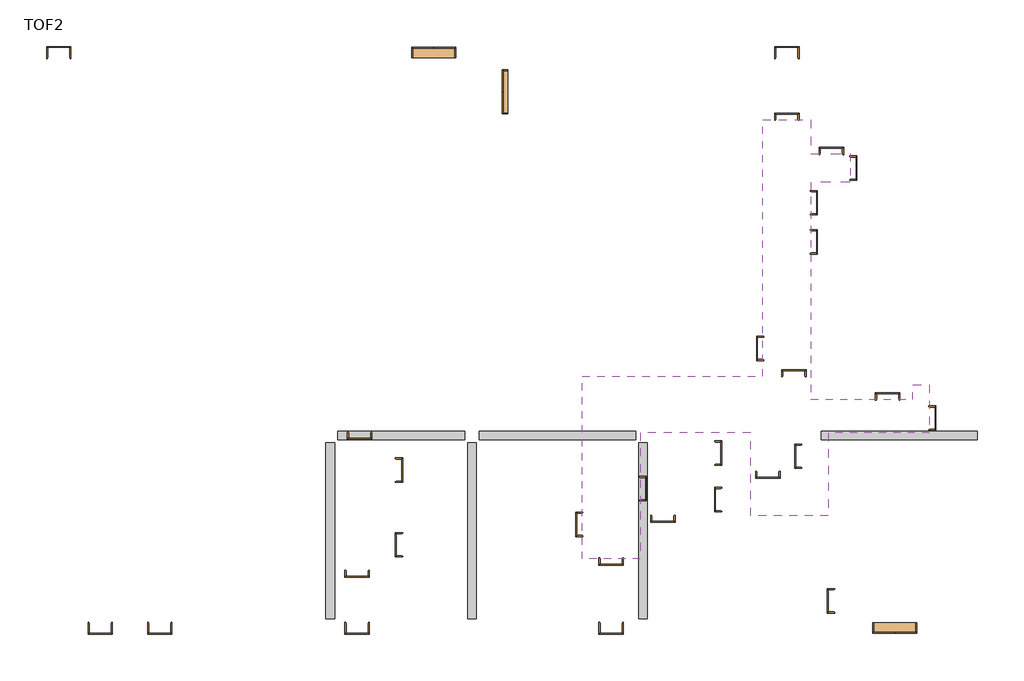
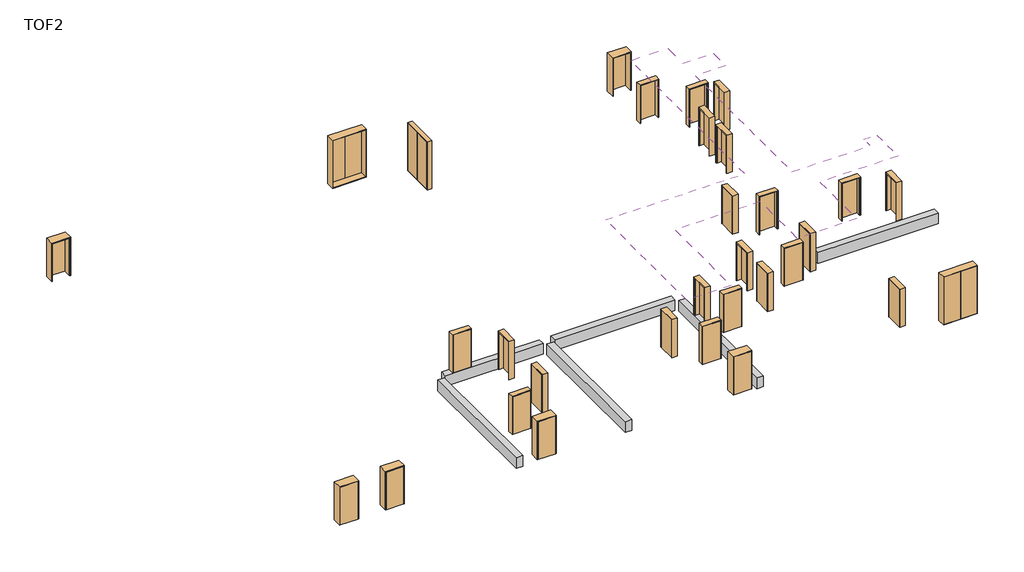
# One storey: 31 doors, 6 beams, 1 covering.
"""IFC4 building model written with IfcOpenShell, lengths in millimetres."""

import ifcopenshell
import ifcopenshell.guid

model = None  # the IFC model being written
_history = None  # IfcOwnerHistory: only IFC2X3 demands one
_inside = {}  # id of a spatial element -> (the spatial element, [elements in it])
_under = {}  # id of a project, library or spatial element -> (it, [spatial elements below it])
_declared = {}  # id of a project -> (the project, [libraries it declares])
_typed = {}  # id of a type object -> (the type object, [elements of that type])
_made_of = {}  # id of a material, layer set ... -> (it, [elements and type objects made of it])


def new_model(schema):
    """Start an empty IFC model of exactly this schema.

    Asked for "IFC4X3", IfcOpenShell would pick the latest addendum, in which some entities
    have other attributes; the version numbers below select the first issue.
    IFC2X3 requires an IfcOwnerHistory on every rooted entity: one is made here for all.
    """
    global model, _history
    if schema == "IFC4X3":
        model = ifcopenshell.file(schema_version=(4, 3, 0, 0))
    else:
        model = ifcopenshell.file(schema=schema)
    _inside.clear()
    _under.clear()
    _declared.clear()
    _typed.clear()
    _made_of.clear()
    _history = None
    if model.schema == "IFC2X3":
        org = make("IfcOrganization", Name="unknown")
        user = make(
            "IfcPersonAndOrganization",
            ThePerson=make("IfcPerson", FamilyName="unknown"),
            TheOrganization=org,
        )
        app = make(
            "IfcApplication",
            ApplicationDeveloper=org,
            Version="unknown",
            ApplicationFullName="unknown",
            ApplicationIdentifier="unknown",
        )
        _history = make(
            "IfcOwnerHistory",
            OwningUser=user,
            OwningApplication=app,
            ChangeAction="ADDED",
            CreationDate=0,
        )
    return model


def make(cls, **values):
    """One entity of the class cls with the attributes given. An attribute that is None is left unset."""
    return model.create_entity(
        cls, **{name: value for name, value in values.items() if value is not None}
    )


def rooted(cls, **values):
    """An entity with a GlobalId (a new one), such as an element, a storey or a relation."""
    return make(cls, GlobalId=ifcopenshell.guid.new(), OwnerHistory=_history, **values)


def si_unit(unit_type, name, prefix=None):
    """IfcSIUnit, for example si_unit("LENGTHUNIT", "METRE", prefix="MILLI")."""
    return make("IfcSIUnit", UnitType=unit_type, Prefix=prefix, Name=name)


def assignment(units):
    """IfcUnitAssignment: the units of a project."""
    return None if units is None else make("IfcUnitAssignment", Units=units)


def point(xyz):
    """IfcCartesianPoint."""
    return None if xyz is None else make("IfcCartesianPoint", Coordinates=xyz)


def direction(xyz):
    """IfcDirection."""
    return None if xyz is None else make("IfcDirection", DirectionRatios=xyz)


def frame(location, z_axis=None, x_axis=None):
    """IfcAxis2Placement3D, a coordinate frame: its origin and axes. An axis left out is left unset."""
    return make(
        "IfcAxis2Placement3D",
        Location=point(location),
        Axis=direction(z_axis),
        RefDirection=direction(x_axis),
    )


def origin():
    """The frame at (0, 0, 0) with its axes left unset."""
    return frame((0.0, 0.0, 0.0))


def origin_with_axes():
    """The frame at (0, 0, 0) with the z axis (0, 0, 1) and the x axis (1, 0, 0) written out."""
    return frame((0.0, 0.0, 0.0), z_axis=(0.0, 0.0, 1.0), x_axis=(1.0, 0.0, 0.0))


def place(relative_to, where):
    """IfcLocalPlacement: puts the frame where relative to a parent placement (None: the world)."""
    return make(
        "IfcLocalPlacement", PlacementRelTo=relative_to, RelativePlacement=where
    )


def context(
    kind, dimensions, precision=None, world=None, true_north=None, identifier=None
):
    """IfcGeometricRepresentationContext, for example the 3D "Model" context."""
    return make(
        "IfcGeometricRepresentationContext",
        ContextIdentifier=identifier,
        ContextType=kind,
        CoordinateSpaceDimension=dimensions,
        Precision=precision,
        WorldCoordinateSystem=world,
        TrueNorth=true_north,
    )


def project(units=None, contexts=None):
    """IfcProject with its units and contexts."""
    return rooted(
        "IfcProject",
        Name="project",
        RepresentationContexts=contexts,
        UnitsInContext=assignment(units),
    )


def spatial(cls, under=None, at=None, **own):
    """A site, building, storey or space (cls), placed at a placement, below another one or the project."""
    s = rooted(cls, ObjectPlacement=at, **own)
    if under is not None:
        _under.setdefault(under.id(), (under, []))[1].append(s)
    return s


def polyline(points):
    """IfcPolyline through the points."""
    return make("IfcPolyline", Points=[point(p) for p in points])


def outline(outer, holes=None, kind="AREA"):
    """IfcArbitraryClosedProfileDef: a profile drawn as a closed curve; with holes, ...WithVoids."""
    if holes is None:
        return make("IfcArbitraryClosedProfileDef", ProfileType=kind, OuterCurve=outer)
    return make(
        "IfcArbitraryProfileDefWithVoids",
        ProfileType=kind,
        OuterCurve=outer,
        InnerCurves=holes,
    )


def extrude(swept, where, along, depth):
    """IfcExtrudedAreaSolid: the profile swept, set in the frame where, extruded along a direction by depth."""
    return make(
        "IfcExtrudedAreaSolid",
        SweptArea=swept,
        Position=where,
        ExtrudedDirection=direction(along),
        Depth=depth,
    )


def faces_of(points, faces, orient=None, outer=None):
    """IfcFace entities. A face is a list of loops; a loop is a list of indices into points, from 0.

    orient and outer hold one flag for each loop. By default every Orientation is true, the
    first loop of a face is its IfcFaceOuterBound and the others are IfcFaceBound.
    """
    made = []
    for i, loops in enumerate(faces):
        bounds = []
        for j, loop in enumerate(loops):
            is_outer = j == 0 if outer is None else outer[i][j]
            bounds.append(
                make(
                    "IfcFaceOuterBound" if is_outer else "IfcFaceBound",
                    Bound=make("IfcPolyLoop", Polygon=[points[k] for k in loop]),
                    Orientation=True if orient is None else orient[i][j],
                )
            )
        made.append(make("IfcFace", Bounds=bounds))
    return made


def faceted_brep(points, faces, orient=None, outer=None, voids=None):
    """IfcFacetedBrep: a solid bounded by flat faces; with voids (closed shells), ...WithVoids."""
    shared = [point(p) for p in points]
    hull = make("IfcClosedShell", CfsFaces=faces_of(shared, faces, orient, outer))
    if voids is None:
        return make("IfcFacetedBrep", Outer=hull)
    return make(
        "IfcFacetedBrepWithVoids",
        Outer=hull,
        Voids=[
            make(cls, CfsFaces=faces_of(shared, fs, o, b)) for cls, fs, o, b in voids
        ],
    )


def shape(context_of_items, identifier, shape_type, items):
    """IfcShapeRepresentation: the items that make up one representation, for example the "Body"."""
    return make(
        "IfcShapeRepresentation",
        ContextOfItems=context_of_items,
        RepresentationIdentifier=identifier,
        RepresentationType=shape_type,
        Items=items,
    )


def source(mapping_origin, context_of_items, identifier, shape_type, items):
    """IfcRepresentationMap: a shape defined once, which mapped items show again and again."""
    return make(
        "IfcRepresentationMap",
        MappingOrigin=mapping_origin,
        MappedRepresentation=shape(context_of_items, identifier, shape_type, items),
    )


def transform(
    local_origin,
    x_axis=None,
    y_axis=None,
    z_axis=None,
    scale=None,
    scale2=None,
    scale3=None,
    uniform=True,
):
    """IfcCartesianTransformationOperator3D, or its non-uniform kind. x_axis, y_axis, z_axis: its Axis1, 2, 3."""
    if uniform:
        return make(
            "IfcCartesianTransformationOperator3D",
            Axis1=direction(x_axis),
            Axis2=direction(y_axis),
            LocalOrigin=point(local_origin),
            Scale=scale,
            Axis3=direction(z_axis),
        )
    return make(
        "IfcCartesianTransformationOperator3DnonUniform",
        Axis1=direction(x_axis),
        Axis2=direction(y_axis),
        LocalOrigin=point(local_origin),
        Scale=scale,
        Axis3=direction(z_axis),
        Scale2=scale2,
        Scale3=scale3,
    )


def mapped(mapping_source, mapping_target):
    """IfcMappedItem: shows the shape of a source again, moved by a transform."""
    return make(
        "IfcMappedItem", MappingSource=mapping_source, MappingTarget=mapping_target
    )


def made_of(thing, what):
    """Note that an element or type object is made of a material, layer set ...; save() writes the relation."""
    if what is not None:
        _made_of.setdefault(what.id(), (what, []))[1].append(thing)
    return thing


def element(
    cls,
    number,
    at=None,
    inside=None,
    cuts=None,
    type_object=None,
    material=None,
    context=None,
    identifier="Body",
    shape_type=None,
    held_by="IfcProductDefinitionShape",
    body=None,
    shapes=None,
    **own,
):
    """One element of the class cls, such as IfcWall. Its Tag is "e" and its number.

    at: its placement. inside: the storey or other place that contains it. cuts: it is an
    opening in that element (IfcRelVoidsElement). A single representation is given by context,
    identifier, shape_type and body (its items); several are given by shapes. held_by: the class
    of the entity that holds the representations. save() writes the other relations.
    """
    e = rooted(cls, Tag="e%d" % number, ObjectPlacement=at, **own)
    if body is not None:
        shapes = [shape(context, identifier, shape_type, body)]
    if shapes is not None:
        e.Representation = make(held_by, Representations=shapes)
    if inside is not None:
        _inside.setdefault(inside.id(), (inside, []))[1].append(e)
    if cuts is not None:
        rooted(
            "IfcRelVoidsElement", RelatingBuildingElement=cuts, RelatedOpeningElement=e
        )
    if type_object is not None:
        _typed.setdefault(type_object.id(), (type_object, []))[1].append(e)
    return made_of(e, material)


def aggregate(whole, parts):
    """IfcRelAggregates: a whole, such as a stair, and the parts it consists of."""
    return rooted("IfcRelAggregates", RelatingObject=whole, RelatedObjects=parts)


def save(model, path):
    """Write the relations noted so far, then the file.

    IfcRelAggregates (storeys below a building ...), IfcRelContainedInSpatialStructure (elements
    in a storey), IfcRelDefinesByType, IfcRelAssociatesMaterial and IfcRelDeclares: one each for
    every whole, place, type object, material and project.
    """
    for whole, parts in _under.values():
        aggregate(whole, parts)
    for where, things in _inside.values():
        rooted(
            "IfcRelContainedInSpatialStructure",
            RelatedElements=things,
            RelatingStructure=where,
        )
    for kind, things in _typed.values():
        rooted("IfcRelDefinesByType", RelatedObjects=things, RelatingType=kind)
    for what, things in _made_of.values():
        rooted("IfcRelAssociatesMaterial", RelatedObjects=things, RelatingMaterial=what)
    for by, libraries in _declared.values():
        rooted("IfcRelDeclares", RelatingContext=by, RelatedDefinitions=libraries)
    model.write(path)


def double_door_steel_634f6038(model_context):
    return source(origin(), model_context, "Body", "SolidModel", [
        extrude(outline(polyline([(880.0, 175.0), (0.0, 175.0), (0.0, 215.0), (880.0, 215.0), (880.0, 175.0)])), frame((0.0, 0.0, 20.0), z_axis=(0.0, 0.0, 1.0), x_axis=(1.0, 0.0, 0.0)), (0.0, 0.0, 1.0), 2660.0),
        extrude(outline(polyline([(0.0, 175.0), (-880.0, 175.0), (-880.0, 215.0), (0.0, 215.0), (0.0, 175.0)])), frame((0.0, 0.0, 20.0), z_axis=(0.0, 0.0, 1.0), x_axis=(1.0, 0.0, 0.0)), (0.0, 0.0, 1.0), 2660.0),
        faceted_brep([(900.0, -215.0, 2700.0), (900.0, 215.0, 2700.0), (-900.0, 215.0, 2700.0), (-900.0, -215.0, 2700.0), (865.0, 175.0, 2665.0), (865.0, -215.0, 2665.0), (-865.0, -215.0, 2665.0), (-865.0, 175.0, 2665.0), (880.0, 215.0, 2680.0), (880.0, 175.0, 2680.0), (-880.0, 175.0, 2680.0), (-880.0, 215.0, 2680.0), (-900.0, 215.0, 0.0), (-900.0, -215.0, 0.0), (-865.0, -215.0, 35.0), (-865.0, 175.0, 35.0), (-880.0, 175.0, 20.0), (-880.0, 215.0, 20.0), (900.0, 215.0, 0.0), (880.0, 215.0, 20.0), (900.0, -215.0, 0.0), (865.0, -215.0, 35.0), (865.0, 175.0, 35.0), (880.0, 175.0, 20.0)], [[[0, 1, 2, 3]], [[4, 5, 6, 7]], [[8, 9, 10, 11]], [[3, 2, 12, 13]], [[7, 6, 14, 15]], [[11, 10, 16, 17]], [[18, 12, 2, 1], [8, 11, 17, 19]], [[13, 12, 18, 20]], [[0, 3, 13, 20], [21, 14, 6, 5]], [[15, 14, 21, 22]], [[23, 16, 10, 9], [4, 7, 15, 22]], [[17, 16, 23, 19]], [[20, 18, 1, 0]], [[22, 21, 5, 4]], [[19, 23, 9, 8]]]),
    ])


def double_door_steel_474d71af(model_context):
    return source(origin(), model_context, "Body", "SolidModel", [
        extrude(outline(polyline([(880.0, 77.0), (0.0, 77.0), (0.0, 117.0), (880.0, 117.0), (880.0, 77.0)])), frame((0.0, 0.0, 20.0), z_axis=(0.0, 0.0, 1.0), x_axis=(1.0, 0.0, 0.0)), (0.0, 0.0, 1.0), 2660.0),
        extrude(outline(polyline([(0.0, 77.0), (-880.0, 77.0), (-880.0, 117.0), (0.0, 117.0), (0.0, 77.0)])), frame((0.0, 0.0, 20.0), z_axis=(0.0, 0.0, 1.0), x_axis=(1.0, 0.0, 0.0)), (0.0, 0.0, 1.0), 2660.0),
        faceted_brep([(900.0, -117.0, 2700.0), (900.0, 117.0, 2700.0), (-900.0, 117.0, 2700.0), (-900.0, -117.0, 2700.0), (865.0, 77.0, 2665.0), (865.0, -117.0, 2665.0), (-865.0, -117.0, 2665.0), (-865.0, 77.0, 2665.0), (880.0, 117.0, 2680.0), (880.0, 77.0, 2680.0), (-880.0, 77.0, 2680.0), (-880.0, 117.0, 2680.0), (-900.0, 117.0, 0.0), (-900.0, -117.0, 0.0), (-865.0, -117.0, 35.0), (-865.0, 77.0, 35.0), (-880.0, 77.0, 20.0), (-880.0, 117.0, 20.0), (900.0, 117.0, 0.0), (880.0, 117.0, 20.0), (900.0, -117.0, 0.0), (865.0, -117.0, 35.0), (865.0, 77.0, 35.0), (880.0, 77.0, 20.0)], [[[0, 1, 2, 3]], [[4, 5, 6, 7]], [[8, 9, 10, 11]], [[3, 2, 12, 13]], [[7, 6, 14, 15]], [[11, 10, 16, 17]], [[18, 12, 2, 1], [8, 11, 17, 19]], [[13, 12, 18, 20]], [[0, 3, 13, 20], [21, 14, 6, 5]], [[15, 14, 21, 22]], [[23, 16, 10, 9], [4, 7, 15, 22]], [[17, 16, 23, 19]], [[20, 18, 1, 0]], [[22, 21, 5, 4]], [[19, 23, 9, 8]]]),
    ])


def single_door_steel_cad2a4f8(model_context):
    return source(origin(), model_context, "Body", "SolidModel", [
        extrude(outline(polyline([(470.0, -245.0), (-470.0, -245.0), (-470.0, -210.0), (470.0, -210.0), (470.0, -245.0)])), origin_with_axes(), (0.0, 0.0, 1.0), 2120.0),
        faceted_brep([(470.0, -245.0, 0.0), (470.0, -210.0, 0.0), (450.0, -210.0, 0.0), (450.0, 210.0, 0.0), (470.0, 210.0, 0.0), (470.0, 245.0, 0.0), (500.0, 245.0, 0.0), (500.0, -245.0, 0.0), (500.0, -245.0, 2150.0), (-500.0, -245.0, 2150.0), (-500.0, -245.0, 0.0), (-470.0, -245.0, 0.0), (-470.0, -245.0, 2120.0), (470.0, -245.0, 2120.0), (500.0, 245.0, 2150.0), (470.0, 245.0, 2120.0), (-470.0, 245.0, 2120.0), (-470.0, 245.0, 0.0), (-500.0, 245.0, 0.0), (-500.0, 245.0, 2150.0), (470.0, 210.0, 2120.0), (450.0, 210.0, 2100.0), (-450.0, 210.0, 2100.0), (-450.0, 210.0, 0.0), (-470.0, 210.0, 0.0), (-470.0, 210.0, 2120.0), (450.0, -210.0, 2100.0), (470.0, -210.0, 2120.0), (-470.0, -210.0, 2120.0), (-470.0, -210.0, 0.0), (-450.0, -210.0, 0.0), (-450.0, -210.0, 2100.0)], [[[0, 1, 2, 3, 4, 5, 6, 7]], [[7, 8, 9, 10, 11, 12, 13, 0]], [[6, 14, 8, 7]], [[5, 15, 16, 17, 18, 19, 14, 6]], [[4, 20, 15, 5]], [[3, 21, 22, 23, 24, 25, 20, 4]], [[2, 26, 21, 3]], [[1, 27, 28, 29, 30, 31, 26, 2]], [[0, 13, 27, 1]], [[12, 11, 29, 28]], [[11, 10, 18, 17, 24, 23, 30, 29]], [[19, 18, 10, 9]], [[25, 24, 17, 16]], [[31, 30, 23, 22]], [[14, 19, 9, 8]], [[20, 25, 16, 15]], [[26, 31, 22, 21]], [[13, 12, 28, 27]]]),
    ])


def single_door_steel_d38beafa(model_context):
    return source(origin(), model_context, "Body", "SolidModel", [
        extrude(outline(polyline([(470.0, 147.0), (470.0, 112.0), (-470.0, 112.0), (-470.0, 147.0), (470.0, 147.0)])), origin_with_axes(), (0.0, 0.0, 1.0), 2120.0),
        faceted_brep([(470.0, 147.0, 0.0), (500.0, 147.0, 0.0), (500.0, -147.0, 0.0), (470.0, -147.0, 0.0), (470.0, -112.0, 0.0), (450.0, -112.0, 0.0), (450.0, 112.0, 0.0), (470.0, 112.0, 0.0), (470.0, 147.0, 2120.0), (-470.0, 147.0, 2120.0), (-470.0, 147.0, 0.0), (-500.0, 147.0, 0.0), (-500.0, 147.0, 2150.0), (500.0, 147.0, 2150.0), (500.0, -147.0, 2150.0), (-500.0, -147.0, 2150.0), (-500.0, -147.0, 0.0), (-470.0, -147.0, 0.0), (-470.0, -147.0, 2120.0), (470.0, -147.0, 2120.0), (470.0, -112.0, 2120.0), (-470.0, -112.0, 2120.0), (-470.0, -112.0, 0.0), (-450.0, -112.0, 0.0), (-450.0, -112.0, 2100.0), (450.0, -112.0, 2100.0), (450.0, 112.0, 2100.0), (-450.0, 112.0, 2100.0), (-450.0, 112.0, 0.0), (-470.0, 112.0, 0.0), (-470.0, 112.0, 2120.0), (470.0, 112.0, 2120.0)], [[[0, 1, 2, 3, 4, 5, 6, 7]], [[1, 0, 8, 9, 10, 11, 12, 13]], [[2, 1, 13, 14]], [[3, 2, 14, 15, 16, 17, 18, 19]], [[4, 3, 19, 20]], [[5, 4, 20, 21, 22, 23, 24, 25]], [[6, 5, 25, 26]], [[7, 6, 26, 27, 28, 29, 30, 31]], [[0, 7, 31, 8]], [[9, 30, 29, 10]], [[10, 29, 28, 23, 22, 17, 16, 11]], [[15, 12, 11, 16]], [[21, 18, 17, 22]], [[27, 24, 23, 28]], [[14, 13, 12, 15]], [[20, 19, 18, 21]], [[26, 25, 24, 27]], [[8, 31, 30, 9]]]),
    ])


def single_door_steel_221a647d(model_context):
    return source(origin(), model_context, "Body", "SolidModel", [
        extrude(outline(polyline([(470.0, -147.0), (-470.0, -147.0), (-470.0, -112.0), (470.0, -112.0), (470.0, -147.0)])), origin_with_axes(), (0.0, 0.0, 1.0), 2120.0),
        faceted_brep([(470.0, -147.0, 0.0), (470.0, -112.0, 0.0), (450.0, -112.0, 0.0), (450.0, 112.0, 0.0), (470.0, 112.0, 0.0), (470.0, 147.0, 0.0), (500.0, 147.0, 0.0), (500.0, -147.0, 0.0), (500.0, -147.0, 2150.0), (-500.0, -147.0, 2150.0), (-500.0, -147.0, 0.0), (-470.0, -147.0, 0.0), (-470.0, -147.0, 2120.0), (470.0, -147.0, 2120.0), (500.0, 147.0, 2150.0), (470.0, 147.0, 2120.0), (-470.0, 147.0, 2120.0), (-470.0, 147.0, 0.0), (-500.0, 147.0, 0.0), (-500.0, 147.0, 2150.0), (470.0, 112.0, 2120.0), (450.0, 112.0, 2100.0), (-450.0, 112.0, 2100.0), (-450.0, 112.0, 0.0), (-470.0, 112.0, 0.0), (-470.0, 112.0, 2120.0), (450.0, -112.0, 2100.0), (470.0, -112.0, 2120.0), (-470.0, -112.0, 2120.0), (-470.0, -112.0, 0.0), (-450.0, -112.0, 0.0), (-450.0, -112.0, 2100.0)], [[[0, 1, 2, 3, 4, 5, 6, 7]], [[7, 8, 9, 10, 11, 12, 13, 0]], [[6, 14, 8, 7]], [[5, 15, 16, 17, 18, 19, 14, 6]], [[4, 20, 15, 5]], [[3, 21, 22, 23, 24, 25, 20, 4]], [[2, 26, 21, 3]], [[1, 27, 28, 29, 30, 31, 26, 2]], [[0, 13, 27, 1]], [[12, 11, 29, 28]], [[11, 10, 18, 17, 24, 23, 30, 29]], [[19, 18, 10, 9]], [[25, 24, 17, 16]], [[31, 30, 23, 22]], [[14, 19, 9, 8]], [[20, 25, 16, 15]], [[26, 31, 22, 21]], [[13, 12, 28, 27]]]),
    ])


def single_door_steel_7afc0ab2(model_context):
    return source(origin(), model_context, "Body", "SolidModel", [
        extrude(outline(polyline([(470.0, 245.0), (470.0, 210.0), (-470.0, 210.0), (-470.0, 245.0), (470.0, 245.0)])), origin_with_axes(), (0.0, 0.0, 1.0), 2120.0),
        faceted_brep([(470.0, 245.0, 0.0), (500.0, 245.0, 0.0), (500.0, -245.0, 0.0), (470.0, -245.0, 0.0), (470.0, -210.0, 0.0), (450.0, -210.0, 0.0), (450.0, 210.0, 0.0), (470.0, 210.0, 0.0), (470.0, 245.0, 2120.0), (-470.0, 245.0, 2120.0), (-470.0, 245.0, 0.0), (-500.0, 245.0, 0.0), (-500.0, 245.0, 2150.0), (500.0, 245.0, 2150.0), (500.0, -245.0, 2150.0), (-500.0, -245.0, 2150.0), (-500.0, -245.0, 0.0), (-470.0, -245.0, 0.0), (-470.0, -245.0, 2120.0), (470.0, -245.0, 2120.0), (470.0, -210.0, 2120.0), (-470.0, -210.0, 2120.0), (-470.0, -210.0, 0.0), (-450.0, -210.0, 0.0), (-450.0, -210.0, 2100.0), (450.0, -210.0, 2100.0), (450.0, 210.0, 2100.0), (-450.0, 210.0, 2100.0), (-450.0, 210.0, 0.0), (-470.0, 210.0, 0.0), (-470.0, 210.0, 2120.0), (470.0, 210.0, 2120.0)], [[[0, 1, 2, 3, 4, 5, 6, 7]], [[1, 0, 8, 9, 10, 11, 12, 13]], [[2, 1, 13, 14]], [[3, 2, 14, 15, 16, 17, 18, 19]], [[4, 3, 19, 20]], [[5, 4, 20, 21, 22, 23, 24, 25]], [[6, 5, 25, 26]], [[7, 6, 26, 27, 28, 29, 30, 31]], [[0, 7, 31, 8]], [[9, 30, 29, 10]], [[10, 29, 28, 23, 22, 17, 16, 11]], [[15, 12, 11, 16]], [[21, 18, 17, 22]], [[27, 24, 23, 28]], [[14, 13, 12, 15]], [[20, 19, 18, 21]], [[26, 25, 24, 27]], [[8, 31, 30, 9]]]),
    ])


model = new_model("IFC4")

# Units and contexts
model_context = context("Model", 3, world=origin())
ifc_project = project(units=[si_unit("LENGTHUNIT", "METRE", prefix="MILLI")], contexts=[model_context])

# Site, building, storey
site = spatial("IfcSite", under=ifc_project)
building = spatial("IfcBuilding", under=site)
storey = spatial("IfcBuildingStorey", under=building, Name="TOF2", Elevation=1150.0)

# Beams
placement = place(None, origin())
element("IfcBeam", 1, ObjectType="RC Beam_Rectangular : H_SB_ACB_TG_B400xH600", at=placement, inside=storey, context=model_context, shape_type="SweptSolid", body=[
    extrude(outline(polyline([(31749.7, 8116.5208589), (32099.7, 8116.5208589), (32099.7, 916.5208589), (31749.7, 916.5208589), (31749.7, 8116.5208589)])), frame((0.0, 0.0, 550.0), z_axis=(0.0, 0.0, 1.0), x_axis=(1.0, 0.0, 0.0)), (0.0, 0.0, 1.0), 600.0),
])
element("IfcBeam", 2, ObjectType="RC Beam_Rectangular : H_SB_ACB_TG_B400xH600", at=placement, inside=storey, context=model_context, shape_type="SweptSolid", body=[
    extrude(outline(polyline([(25949.7, 8116.5208589), (26299.7, 8116.5208589), (26299.7, 916.5208589), (25949.7, 916.5208589), (25949.7, 8116.5208589)])), frame((0.0, 0.0, 550.0), z_axis=(0.0, 0.0, 1.0), x_axis=(1.0, 0.0, 0.0)), (0.0, 0.0, 1.0), 600.0),
])
element("IfcBeam", 3, ObjectType="RC Beam_Rectangular : H_SB_ACB_TG_B400xH600", at=placement, inside=storey, context=model_context, shape_type="SweptSolid", body=[
    extrude(outline(polyline([(38749.7, 8116.5208589), (39099.7, 8116.5208589), (39099.7, 916.5208589), (38749.7, 916.5208589), (38749.7, 8116.5208589)])), frame((0.0, 0.0, 550.0), z_axis=(0.0, 0.0, 1.0), x_axis=(1.0, 0.0, 0.0)), (0.0, 0.0, 1.0), 600.0),
])
element("IfcBeam", 4, ObjectType="RC Beam_Rectangular : H_SB_ACB_TG_B400xH600", at=placement, inside=storey, context=model_context, shape_type="SweptSolid", body=[
    extrude(outline(polyline([(26424.7, 8241.5208589), (26424.7, 8591.5208589), (31624.7, 8591.5208589), (31624.7, 8241.5208589), (26424.7, 8241.5208589)])), frame((0.0, 0.0, 550.0), z_axis=(0.0, 0.0, 1.0), x_axis=(1.0, 0.0, 0.0)), (0.0, 0.0, 1.0), 600.0),
])
element("IfcBeam", 5, ObjectType="RC Beam_Rectangular : H_SB_ACB_TG_B400xH600", at=placement, inside=storey, context=model_context, shape_type="SweptSolid", body=[
    extrude(outline(polyline([(32224.7, 8241.5208589), (32224.7, 8591.5208589), (38624.7, 8591.5208589), (38624.7, 8241.5208589), (32224.7, 8241.5208589)])), frame((0.0, 0.0, 550.0), z_axis=(0.0, 0.0, 1.0), x_axis=(1.0, 0.0, 0.0)), (0.0, 0.0, 1.0), 600.0),
])
element("IfcBeam", 6, ObjectType="RC Beam_Rectangular : H_SB_ACB_TG_B400xH600", at=placement, inside=storey, context=model_context, shape_type="SweptSolid", body=[
    extrude(outline(polyline([(46224.7, 8241.5208589), (46224.7, 8591.5208589), (52624.7, 8591.5208589), (52624.7, 8241.5208589), (46224.7, 8241.5208589)])), frame((0.0, 0.0, 550.0), z_axis=(0.0, 0.0, 1.0), x_axis=(1.0, 0.0, 0.0)), (0.0, 0.0, 1.0), 600.0),
])

# Covering
element("IfcCovering", 7, ObjectType="CE741_Acoustic Tiled Ceiling System_600x600x9t_T_bar", at=placement, inside=storey, context=model_context, shape_type="SweptSolid", body=[
    extrude(outline(polyline([(46507.7, 8533.5208589), (46507.7, 5130.5208589), (43341.7, 5130.5208589), (43341.7, 8533.5208589), (38807.7, 8533.5208589), (38807.7, 3380.5208589), (36441.7, 3380.5208589), (36441.7, 10849.5208589), (43841.7, 10849.5208589), (43841.7, 21352.5208589), (45807.7, 21352.5208589), (45807.7, 19949.5208589), (47424.7, 19949.5208589), (47424.7, 18783.5208589), (45807.7, 18783.5208589), (45807.7, 9899.5208589), (49977.7, 9899.5208589), (49977.7, 10499.5208589), (50660.7, 10499.5208589), (50660.7, 8533.5208589), (46507.7, 8533.5208589)])), frame((0.0, 0.0, 4850.0), z_axis=(0.0, 0.0, 1.0), x_axis=(1.0, 0.0, 0.0)), (0.0, 0.0, 1.0), 9.0),
])

# Doors
double_door_steel_shape = double_door_steel_634f6038(model_context)
element("IfcDoor", 8, ObjectType="Double Door_Steel : H_DR_AMB_Double Door_Steel_W1800xH2700", at=placement, inside=storey, context=model_context, shape_type="MappedRepresentation", body=[
    mapped(double_door_steel_shape, transform((30357.7, 24101.5208589, 1150.0), x_axis=(1.0, 0.0, 0.0), y_axis=(0.0, 1.0, 0.0), z_axis=(0.0, 0.0, 1.0))),
])
element("IfcDoor", 9, ObjectType="Double Door_Steel : H_DR_AMB_Double Door_Steel_W1800xH2700", at=placement, inside=storey, context=model_context, shape_type="MappedRepresentation", body=[
    mapped(double_door_steel_shape, transform((49241.7, 531.5208589, 1150.0), x_axis=(-1.0, 0.0, 0.0), y_axis=(0.0, -1.0, 0.0), z_axis=(0.0, 0.0, 1.0))),
])
double_door_steel_2_shape = double_door_steel_474d71af(model_context)
element("IfcDoor", 10, ObjectType="Double Door_Steel : H_DR_AMB_Double Door_Steel_W1800xH2700", at=placement, inside=storey, context=model_context, shape_type="MappedRepresentation", body=[
    mapped(double_door_steel_2_shape, transform((33274.7, 22486.5208589, 1150.0), x_axis=(0.0, 1.0, 0.0), y_axis=(-1.0, 0.0, 0.0), z_axis=(0.0, 0.0, 1.0))),
])
single_door_steel_shape = single_door_steel_cad2a4f8(model_context)
element("IfcDoor", 11, ObjectType="Single Door_Steel : H_DR_AMB_Single Door_Steel_W1000xH2150", at=placement, inside=storey, context=model_context, shape_type="MappedRepresentation", body=[
    mapped(single_door_steel_shape, transform((15007.7, 24101.5208589, 1150.0), x_axis=(-1.0, 0.0, 0.0), y_axis=(0.0, -1.0, 0.0), z_axis=(0.0, 0.0, 1.0))),
])
element("IfcDoor", 12, ObjectType="Single Door_Steel : H_DR_AMB_Single Door_Steel_W1000xH2150", at=placement, inside=storey, context=model_context, shape_type="MappedRepresentation", body=[
    mapped(single_door_steel_shape, transform((44824.7, 24101.5208589, 1150.0), x_axis=(-1.0, 0.0, 0.0), y_axis=(0.0, -1.0, 0.0), z_axis=(0.0, 0.0, 1.0))),
])
element("IfcDoor", 13, ObjectType="Single Door_Steel : H_DR_AMB_Single Door_Steel_W1000xH2150", at=placement, inside=storey, context=model_context, shape_type="MappedRepresentation", body=[
    mapped(single_door_steel_shape, transform((19141.7, 531.5208589, 1150.0), x_axis=(1.0, 0.0, 0.0), y_axis=(0.0, 1.0, 0.0), z_axis=(0.0, 0.0, 1.0))),
])
element("IfcDoor", 14, ObjectType="Single Door_Steel : H_DR_AMB_Single Door_Steel_W1000xH2150", at=placement, inside=storey, context=model_context, shape_type="MappedRepresentation", body=[
    mapped(single_door_steel_shape, transform((27224.7, 531.5208589, 1150.0), x_axis=(1.0, 0.0, 0.0), y_axis=(0.0, 1.0, 0.0), z_axis=(0.0, 0.0, 1.0))),
])
single_door_steel_2_shape = single_door_steel_d38beafa(model_context)
element("IfcDoor", 15, ObjectType="Single Door_Steel : H_DR_AMB_Single Door_Steel_W1000xH2150", at=placement, inside=storey, context=model_context, shape_type="MappedRepresentation", body=[
    mapped(single_door_steel_2_shape, transform((43724.7, 11983.5208589, 1150.0), x_axis=(0.0, 1.0, 0.0), y_axis=(-1.0, 0.0, 0.0), z_axis=(0.0, 0.0, 1.0))),
])
element("IfcDoor", 16, ObjectType="Single Door_Steel : H_DR_AMB_Single Door_Steel_W1000xH2150", at=placement, inside=storey, context=model_context, shape_type="MappedRepresentation", body=[
    mapped(single_door_steel_2_shape, transform((46641.7, 20066.5208589, 1150.0), x_axis=(1.0, 0.0, 0.0), y_axis=(0.0, 1.0, 0.0), z_axis=(0.0, 0.0, 1.0))),
])
element("IfcDoor", 17, ObjectType="Single Door_Steel : H_DR_AMB_Single Door_Steel_W1000xH2150", at=placement, inside=storey, context=model_context, shape_type="MappedRepresentation", body=[
    mapped(single_door_steel_2_shape, transform((45924.7, 17949.5208589, 1150.0), x_axis=(0.0, -1.0, 0.0), y_axis=(1.0, 0.0, 0.0), z_axis=(0.0, 0.0, 1.0))),
])
element("IfcDoor", 18, ObjectType="Single Door_Steel : H_DR_AMB_Single Door_Steel_W1000xH2150", at=placement, inside=storey, context=model_context, shape_type="MappedRepresentation", body=[
    mapped(single_door_steel_2_shape, transform((45924.7, 16350.3721317, 1150.0), x_axis=(0.0, -1.0, 0.0), y_axis=(1.0, 0.0, 0.0), z_axis=(0.0, 0.0, 1.0))),
])
element("IfcDoor", 19, ObjectType="Single Door_Steel : H_DR_AMB_Single Door_Steel_W1000xH2150", at=placement, inside=storey, context=model_context, shape_type="MappedRepresentation", body=[
    mapped(single_door_steel_2_shape, transform((48943.7, 10016.5208589, 1150.0), x_axis=(1.0, 0.0, 0.0), y_axis=(0.0, 1.0, 0.0), z_axis=(0.0, 0.0, 1.0))),
])
element("IfcDoor", 20, ObjectType="Single Door_Steel : H_DR_AMB_Single Door_Steel_W1000xH2150", at=placement, inside=storey, context=model_context, shape_type="MappedRepresentation", body=[
    mapped(single_door_steel_2_shape, transform((36324.7, 4780.5208589, 1150.0), x_axis=(0.0, 1.0, 0.0), y_axis=(-1.0, 0.0, 0.0), z_axis=(0.0, 0.0, 1.0))),
])
element("IfcDoor", 21, ObjectType="Single Door_Steel : H_DR_AMB_Single Door_Steel_W1000xH2150", at=placement, inside=storey, context=model_context, shape_type="MappedRepresentation", body=[
    mapped(single_door_steel_2_shape, transform((37624.7, 3263.5208589, 1150.0), x_axis=(-1.0, 0.0, 0.0), y_axis=(0.0, -1.0, 0.0), z_axis=(0.0, 0.0, 1.0))),
])
element("IfcDoor", 22, ObjectType="Single Door_Steel : H_DR_AMB_Single Door_Steel_W1000xH2150", at=placement, inside=storey, context=model_context, shape_type="MappedRepresentation", body=[
    mapped(single_door_steel_2_shape, transform((46624.7, 1646.5208589, 1150.0), x_axis=(0.0, 1.0, 0.0), y_axis=(-1.0, 0.0, 0.0), z_axis=(0.0, 0.0, 1.0))),
])
element("IfcDoor", 23, ObjectType="Single Door_Steel : H_DR_AMB_Single Door_Steel_W1000xH2150", at=placement, inside=storey, context=model_context, shape_type="MappedRepresentation", body=[
    mapped(single_door_steel_2_shape, transform((45292.8778017, 7571.4042881, 1150.0), x_axis=(0.0, 1.0, 0.0), y_axis=(-1.0, 0.0, 0.0), z_axis=(0.0, 0.0, 1.0))),
])
element("IfcDoor", 24, ObjectType="Single Door_Steel : H_DR_AMB_Single Door_Steel_W1000xH2150", at=placement, inside=storey, context=model_context, shape_type="MappedRepresentation", body=[
    mapped(single_door_steel_2_shape, transform((28941.7, 6999.5208589, 1150.0), x_axis=(0.0, -1.0, 0.0), y_axis=(1.0, 0.0, 0.0), z_axis=(0.0, 0.0, 1.0))),
])
element("IfcDoor", 25, ObjectType="Single Door_Steel : H_DR_AMB_Single Door_Steel_W1000xH2150", at=placement, inside=storey, context=model_context, shape_type="MappedRepresentation", body=[
    mapped(single_door_steel_2_shape, transform((38924.7, 6246.5208589, 1150.0), x_axis=(0.0, -1.0, 0.0), y_axis=(1.0, 0.0, 0.0), z_axis=(0.0, 0.0, 1.0))),
])
element("IfcDoor", 26, ObjectType="Single Door_Steel : H_DR_AMB_Single Door_Steel_W1000xH2150", at=placement, inside=storey, context=model_context, shape_type="MappedRepresentation", body=[
    mapped(single_door_steel_2_shape, transform((42007.7, 5792.3649029, 1150.0), x_axis=(0.0, 1.0, 0.0), y_axis=(-1.0, 0.0, 0.0), z_axis=(0.0, 0.0, 1.0))),
])
element("IfcDoor", 27, ObjectType="Single Door_Steel : H_DR_AMB_Single Door_Steel_W1000xH2150", at=placement, inside=storey, context=model_context, shape_type="MappedRepresentation", body=[
    mapped(single_door_steel_2_shape, transform((42007.7, 7699.5208589, 1150.0), x_axis=(0.0, -1.0, 0.0), y_axis=(1.0, 0.0, 0.0), z_axis=(0.0, 0.0, 1.0))),
])
single_door_steel_3_shape = single_door_steel_221a647d(model_context)
element("IfcDoor", 28, ObjectType="Single Door_Steel : H_DR_AMB_Single Door_Steel_W1000xH2150", at=placement, inside=storey, context=model_context, shape_type="MappedRepresentation", body=[
    mapped(single_door_steel_3_shape, transform((27324.7, 8416.5208589, 1150.0), x_axis=(1.0, 0.0, 0.0), y_axis=(0.0, 1.0, 0.0), z_axis=(0.0, 0.0, 1.0))),
])
element("IfcDoor", 29, ObjectType="Single Door_Steel : H_DR_AMB_Single Door_Steel_W1000xH2150", at=placement, inside=storey, context=model_context, shape_type="MappedRepresentation", body=[
    mapped(single_door_steel_3_shape, transform((44824.7, 21469.5208589, 1150.0), x_axis=(-1.0, 0.0, 0.0), y_axis=(0.0, -1.0, 0.0), z_axis=(0.0, 0.0, 1.0))),
])
element("IfcDoor", 30, ObjectType="Single Door_Steel : H_DR_AMB_Single Door_Steel_W1000xH2150", at=placement, inside=storey, context=model_context, shape_type="MappedRepresentation", body=[
    mapped(single_door_steel_3_shape, transform((47541.7, 19366.5208589, 1150.0), x_axis=(0.0, 1.0, 0.0), y_axis=(-1.0, 0.0, 0.0), z_axis=(0.0, 0.0, 1.0))),
])
element("IfcDoor", 31, ObjectType="Single Door_Steel : H_DR_AMB_Single Door_Steel_W1000xH2150", at=placement, inside=storey, context=model_context, shape_type="MappedRepresentation", body=[
    mapped(single_door_steel_3_shape, transform((50777.7, 9133.5208589, 1150.0), x_axis=(0.0, 1.0, 0.0), y_axis=(-1.0, 0.0, 0.0), z_axis=(0.0, 0.0, 1.0))),
])
element("IfcDoor", 32, ObjectType="Single Door_Steel : H_DR_AMB_Single Door_Steel_W1000xH2150", at=placement, inside=storey, context=model_context, shape_type="MappedRepresentation", body=[
    mapped(single_door_steel_3_shape, transform((45107.7, 10966.5208589, 1150.0), x_axis=(-1.0, 0.0, 0.0), y_axis=(0.0, -1.0, 0.0), z_axis=(0.0, 0.0, 1.0))),
])
element("IfcDoor", 33, ObjectType="Single Door_Steel : H_DR_AMB_Single Door_Steel_W1000xH2150", at=placement, inside=storey, context=model_context, shape_type="MappedRepresentation", body=[
    mapped(single_door_steel_3_shape, transform((28941.7, 3946.5208589, 1150.0), x_axis=(0.0, -1.0, 0.0), y_axis=(1.0, 0.0, 0.0), z_axis=(0.0, 0.0, 1.0))),
])
element("IfcDoor", 34, ObjectType="Single Door_Steel : H_DR_AMB_Single Door_Steel_W1000xH2150", at=placement, inside=storey, context=model_context, shape_type="MappedRepresentation", body=[
    mapped(single_door_steel_3_shape, transform((27224.7, 2763.5208589, 1150.0), x_axis=(1.0, 0.0, 0.0), y_axis=(0.0, 1.0, 0.0), z_axis=(0.0, 0.0, 1.0))),
])
element("IfcDoor", 35, ObjectType="Single Door_Steel : H_DR_AMB_Single Door_Steel_W1000xH2150", at=placement, inside=storey, context=model_context, shape_type="MappedRepresentation", body=[
    mapped(single_door_steel_3_shape, transform((44041.7, 6816.5208589, 1150.0), x_axis=(1.0, 0.0, 0.0), y_axis=(0.0, 1.0, 0.0), z_axis=(0.0, 0.0, 1.0))),
])
element("IfcDoor", 36, ObjectType="Single Door_Steel : H_DR_AMB_Single Door_Steel_W1000xH2150", at=placement, inside=storey, context=model_context, shape_type="MappedRepresentation", body=[
    mapped(single_door_steel_3_shape, transform((39741.7, 5013.5208589, 1150.0), x_axis=(1.0, 0.0, 0.0), y_axis=(0.0, 1.0, 0.0), z_axis=(0.0, 0.0, 1.0))),
])
single_door_steel_4_shape = single_door_steel_7afc0ab2(model_context)
element("IfcDoor", 37, ObjectType="Single Door_Steel : H_DR_AMB_Single Door_Steel_W1000xH2150", at=placement, inside=storey, context=model_context, shape_type="MappedRepresentation", body=[
    mapped(single_door_steel_4_shape, transform((16707.7, 531.5208589, 1150.0), x_axis=(-1.0, 0.0, 0.0), y_axis=(0.0, -1.0, 0.0), z_axis=(0.0, 0.0, 1.0))),
])
element("IfcDoor", 38, ObjectType="Single Door_Steel : H_DR_AMB_Single Door_Steel_W1000xH2150", at=placement, inside=storey, context=model_context, shape_type="MappedRepresentation", body=[
    mapped(single_door_steel_4_shape, transform((37624.7, 531.5208589, 1150.0), x_axis=(-1.0, 0.0, 0.0), y_axis=(0.0, -1.0, 0.0), z_axis=(0.0, 0.0, 1.0))),
])

save(model, "model.ifc")

# Revit data of these elements
# Type "RC Beam_Rectangular : H_SB_ACB_TG_B400xH600"
#   중앙부 하부근 = ""
#   중앙부 상부근 = ""
#   중앙부 보조근 = ""
#   중앙부 늑근 = ""
#   외단부 하부근 = ""
#   외단부 상부근 = ""
#   외단부 보조근 = ""
#   외단부 늑근 = ""
#   부호 = "TG2"
#   내단부 하부근 = ""
#   내단부 상부근 = ""
#   내단부 보조근 = ""
#   내단부 늑근 = ""
#   ALL 하부근 = "3-D20"
#   ALL 상부근 = "4-D20"
#   ALL 보조근 = ""
#   ALL 늑근 = "2-D10 @120"
#   Width = 350.000 mm
#   Height = 600.000 mm
#   Length [instance default] = 1524.000 mm
#   b = 350.000 mm
#   h = 600.000 mm
#   hec_material3 [instance default] = none
#   hec_material2 [instance default] = none
#   hec_material1 [instance default] = none
#   Structural Material [instance default] = none
#   Assembly Code = ""
# Type "CE741_Acoustic Tiled Ceiling System_600x600x9t_T_bar"
#   built-in parameter 1002203 = 1 (stored number, unit not read)
#   built-in parameter 1002202 = 1 (stored number, unit not read)
#   Layers, outside or top first: 9.000 mm no material (function 4)
# Type "Double Door_Steel : H_DR_AMB_Double Door_Steel_W1800xH2700"
#   Type Mark = "363"
#   프레임 = ""
#   철물 = ""
#   유리/마감 = ""
#   위치/개소 = ""
#   부호 = "1/SD"
#   문번호 = ""
#   문기호 = "SD"
#   Analytic Construction = "<None>"
#   Height = 2700.000 mm
#   Width = 1800.000 mm
#   Define Thermal Properties by = 1
#   문 틀 = none
#   문 = none
#   Function = (empty or 0)
#   Assembly Code = ""
#   Wall Closure = (empty or 0)
# Type "Single Door_Steel : H_DR_AMB_Single Door_Steel_W1000xH2150"
#   Type Mark = "364"
#   Analytic Construction = "<None>"
#   프레임 투영 외부. = 25.000 mm
#   프레임 투영 내부. = 25.000 mm
#   프레임 폭 = 75.000 mm
#   Height = 2150.000 mm
#   Width = 1000.000 mm
#   Define Thermal Properties by = 1
#   문 패널 = none
#   문 프레임 = none
#   Function = (empty or 0)
#   Wall Closure = (empty or 0)
# Elements 1, 2, 3, 4, 5, 6 (IfcBeam, "RC Beam_Rectangular : H_SB_ACB_TG_B400xH600")
#   hec_material3 = none
#   hec_material2 = none
#   hec_material1 = none
#   Structural Material = none
#   Phase Created = New Construction
# Element 7 (IfcCovering, "CE741_Acoustic Tiled Ceiling System_600x600x9t_T_bar")
#   Height Offset From Level = 3700.000 mm
#   Phase Created = New Construction
# Elements 8, 9, 10 (IfcDoor, "Double Door_Steel : H_DR_AMB_Double Door_Steel_W1800xH2700")
#   Phase Created = New Construction
# Elements 11, 12, 13, 14, 15, 16, 17, 18, 19, 20, 21, 22, 23, 24, 25, 26, 27, 28, 29, 30, 31, 32, 33, 34, 35, 36, 37, 38 (IfcDoor, "Single Door_Steel : H_DR_AMB_Single Door_Steel_W1000xH2150")
#   Phase Created = New Construction
# Room at (42616.2, 7496.521) mm, phase "New Construction", upper level "TOC", upper offset 6500.000 mm, lower offset -1000.000 mm
#   Comments = ""
#   Number = "127"
#   Name = "SHOWER ROOM"
#   Floor Finish Style Name = "Non-Slip Unglazed Ceramic Tile on Screed + Liquid Waterproofing"
#   Floor Finish Ref. = ""
#   Floor-Base Material = "Concrete Slab"
#   Floor Finish-1 = "Screed"
#   Floor Finish-2 = "Liquid Waterproofing"
#   Floor Finish-3 = "Ceramic Tile"
#   Floor Finish-4 = ""
#   Base Finish Style Name = "Epoxy Paint"
#   Base Finish Ref. = ""
#   Base-Base Material = "Concrete Wall\n/ Masonry Wall \n/ Dry Wall"
#   Base Finish-1 = ""
#   Base Finish-2 = ""
#   Base Finish-3 = "Epoxy Paint"
#   Base Finish-4 = ""
#   Wall Finish-1 = "Glazed Ceramic Tile on Cement Plaster"
#   Wall Finish-2 = "No Ceiling\nFull Height"
#   Wall Finish-3 = "Concrete Wall\n/ Masonry Wall"
#   Wall Finish-4 = "Plastering (Tile Workì í¬í¨)"
#   Ceiling Finish Style Name = "Suspended Moisture Resistant Tiled Ceiling (T-Bar)"
#   Ceiling Finish Ref. = "600x600\nT bar"
#   Ceiling-Base Material = "Concrete Slab"
#   Ceiling Finish-1 = ""
#   Ceiling Finish-2 = ""
#   Ceiling Finish-3 = "Moisture Resistant Tiled Ceiling System (T-Bar)"
#   Ceiling Finish-4 = ""
#   H_Room L = 1800.000 mm
#   H_Room W = 1200.000 mm
#   H_Room H or CH = 7300.000 mm
#   Floor Finish Style No = F31B
#   Base Finish Style No = B03
#   Wall Finish Style No = W32C
#   Ceiling Finish Style No = C96A
# Room at (42616.2, 5955.021) mm, phase "New Construction", upper level "TOC", upper offset 6500.000 mm, lower offset -1000.000 mm
#   Comments = ""
#   Number = "128"
#   Name = "EWH ROOM"
#   Floor Finish Style Name = "Non-Slip Unglazed Ceramic Tile on Screed"
#   Floor Finish Ref. = ""
#   Floor-Base Material = "Concrete Slab"
#   Floor Finish-1 = "Screed"
#   Floor Finish-2 = ""
#   Floor Finish-3 = "Ceramic Tile"
#   Floor Finish-4 = ""
#   Base Finish Style Name = "Epoxy Paint"
#   Base Finish Ref. = ""
#   Base-Base Material = "Concrete Wall\n/ Masonry Wall \n/ Dry Wall"
#   Base Finish-1 = ""
#   Base Finish-2 = ""
#   Base Finish-3 = "Epoxy Paint"
#   Base Finish-4 = ""
#   Wall Finish-1 = "Acrylic Emulsion Paint on Cement Plaster"
#   Wall Finish-2 = "T13 Plaster"
#   Wall Finish-3 = "Masonry Wall"
#   Wall Finish-4 = "Plastering"
#   Ceiling Finish Style Name = "Suspended Acoustic Tiled Ceiling (T-Bar)"
#   Ceiling Finish Ref. = "600x600\nT Bar"
#   Ceiling-Base Material = "Concrete Slab"
#   Ceiling Finish-1 = ""
#   Ceiling Finish-2 = ""
#   Ceiling Finish-3 = "Acoustic Tiled Ceiling System (T-Bar)"
#   Ceiling Finish-4 = ""
#   H_Room L = 1500.000 mm
#   H_Room W = 1200.000 mm
#   H_Room H or CH = 7300.000 mm
#   Floor Finish Style No = F31A
#   Base Finish Style No = B03
#   Wall Finish Style No = W01B
#   Ceiling Finish Style No = C95A
# Room at (30341.7, 6590.021) mm, phase "New Construction", upper level "TOC", upper offset 6500.000 mm, lower offset -1000.000 mm
#   Comments = ""
#   Number = "113"
#   Name = "STORE"
#   Floor Finish Style Name = "Vinyl Tile on Screed"
#   Floor Finish Ref. = ""
#   Floor-Base Material = "Concrete Slab"
#   Floor Finish-1 = "Screed"
#   Floor Finish-2 = ""
#   Floor Finish-3 = "Vinyl Tile"
#   Floor Finish-4 = ""
#   Base Finish Style Name = "Coved Vinyl Tile"
#   Base Finish Ref. = ""
#   Base-Base Material = "Concrete Wall\n/ Masonry Wall"
#   Base Finish-1 = ""
#   Base Finish-2 = ""
#   Base Finish-3 = "Vinyl Tile"
#   Base Finish-4 = ""
#   Wall Finish-1 = "Acrylic Emulsion Paint on Cement Plaster"
#   Wall Finish-2 = "T13 Plaster"
#   Wall Finish-3 = "Masonry Wall"
#   Wall Finish-4 = "Plastering"
#   Ceiling Finish Style Name = "Suspended Acoustic Tiled Ceiling (T-Bar)"
#   Ceiling Finish Ref. = "600x600\nT Bar"
#   Ceiling-Base Material = "Concrete Slab"
#   Ceiling Finish-1 = ""
#   Ceiling Finish-2 = ""
#   Ceiling Finish-3 = "Acoustic Tiled Ceiling System (T-Bar)"
#   Ceiling Finish-4 = ""
#   H_Room L = 3600.000 mm
#   H_Room W = 2700.000 mm
#   H_Room H or CH = 6300.000 mm
#   Floor Finish Style No = F34A
#   Base Finish Style No = B35A
#   Wall Finish Style No = W01B
#   Ceiling Finish Style No = C95A
# Room at (30341.7, 2647.521) mm, phase "New Construction", upper level "TOC", upper offset 6500.000 mm, lower offset -1000.000 mm
#   Comments = ""
#   Number = "115"
#   Name = "TELECOMS ROOM"
#   Floor Finish Style Name = "Vinyl Tile on Screed"
#   Floor Finish Ref. = ""
#   Floor-Base Material = "Concrete Slab"
#   Floor Finish-1 = "Screed"
#   Floor Finish-2 = ""
#   Floor Finish-3 = "Vinyl Tile"
#   Floor Finish-4 = ""
#   Base Finish Style Name = "Coved Vinyl Tile"
#   Base Finish Ref. = ""
#   Base-Base Material = "Concrete Wall\n/ Masonry Wall"
#   Base Finish-1 = ""
#   Base Finish-2 = ""
#   Base Finish-3 = "Vinyl Tile"
#   Base Finish-4 = ""
#   Wall Finish-1 = "2 Coats of Non-Conductive & Fire Retardant White Color Paint on Thk.13 Cement Plaster"
#   Wall Finish-2 = ""
#   Wall Finish-3 = ""
#   Wall Finish-4 = ""
#   Ceiling Finish Style Name = "Acrylic Emulsion Paint on Fair Faced Concrete"
#   Ceiling Finish Ref. = ""
#   Ceiling-Base Material = "Concrete Slab"
#   Ceiling Finish-1 = ""
#   Ceiling Finish-2 = ""
#   Ceiling Finish-3 = "Acrylic Emulsion Paint"
#   Ceiling Finish-4 = ""
#   H_Room L = 4200.000 mm
#   H_Room W = 2700.000 mm
#   H_Room H or CH = 6300.000 mm
#   Floor Finish Style No = F34A
#   Base Finish Style No = B35A
#   Wall Finish Style No = W11
#   Ceiling Finish Style No = C01
# Room at (27624.7, 5590.021) mm, phase "New Construction", upper level "TOC", upper offset 6500.000 mm, lower offset -1000.000 mm
#   Comments = ""
#   Number = "116"
#   Name = "CORRIDOR"
#   Floor Finish Style Name = "Vinyl Tile on Screed"
#   Floor Finish Ref. = ""
#   Floor-Base Material = "Concrete Slab"
#   Floor Finish-1 = "Screed"
#   Floor Finish-2 = ""
#   Floor Finish-3 = "Vinyl Tile"
#   Floor Finish-4 = ""
#   Base Finish Style Name = "Coved Vinyl Tile"
#   Base Finish Ref. = ""
#   Base-Base Material = "Concrete Wall\n/ Masonry Wall"
#   Base Finish-1 = ""
#   Base Finish-2 = ""
#   Base Finish-3 = "Vinyl Tile"
#   Base Finish-4 = ""
#   Wall Finish-1 = "Acrylic Emulsion Paint on Cement Plaster"
#   Wall Finish-2 = "T13 Plaster"
#   Wall Finish-3 = "Masonry Wall"
#   Wall Finish-4 = "Plastering"
#   Ceiling Finish Style Name = "Suspended Acoustic Tiled Ceiling (T-Bar)"
#   Ceiling Finish Ref. = "600x600\nT Bar"
#   Ceiling-Base Material = "Concrete Slab"
#   Ceiling Finish-1 = ""
#   Ceiling Finish-2 = ""
#   Ceiling Finish-3 = "Acoustic Tiled Ceiling System (T-Bar)"
#   Ceiling Finish-4 = ""
#   H_Room L = 5600.000 mm
#   H_Room W = 2600.000 mm
#   H_Room H or CH = 6300.000 mm
#   Floor Finish Style No = F34A
#   Base Finish Style No = B35A
#   Wall Finish Style No = W01B
#   Ceiling Finish Style No = C95A
# Room at (27624.7, 1647.521) mm, phase "New Construction", upper level "TOC", upper offset 6500.000 mm, lower offset -1000.000 mm
#   Comments = ""
#   Number = "117"
#   Name = "AIR LOCK"
#   Floor Finish Style Name = "Vinyl Tile on Screed + Matwell"
#   Base Finish Style Name = "Coved Vinyl Tile"
#   Base Finish Ref. = ""
#   Base-Base Material = "Concrete Wall\n/ Masonry Wall"
#   Base Finish-1 = ""
#   Base Finish-2 = ""
#   Base Finish-3 = "Vinyl Tile"
#   Base Finish-4 = ""
#   Wall Finish-1 = "Acrylic Emulsion Paint on Cement Plaster"
#   Wall Finish-2 = "T13 Plaster"
#   Wall Finish-3 = "Masonry Wall"
#   Wall Finish-4 = "Plastering"
#   Ceiling Finish Style Name = "Suspended Acoustic Tiled Ceiling (T-Bar)"
#   Ceiling Finish Ref. = "600x600\nT Bar"
#   Ceiling-Base Material = "Concrete Slab"
#   Ceiling Finish-1 = ""
#   Ceiling Finish-2 = ""
#   Ceiling Finish-3 = "Acoustic Tiled Ceiling System (T-Bar)"
#   Ceiling Finish-4 = ""
#   H_Room L = 2200.000 mm
#   H_Room W = 2600.000 mm
#   H_Room H or CH = 6300.000 mm
#   Floor Finish Style No = F34A-1
#   Base Finish Style No = B35A
#   Wall Finish Style No = W01B
#   Ceiling Finish Style No = C95A
# Room at (49467.2, 12091.521) mm, phase "New Construction", upper level "TOC", upper offset 6500.000 mm, lower offset -1000.000 mm
#   Comments = ""
#   Number = "111"
#   Name = "PRAYER ROOM"
#   Floor Finish Style Name = "Carpet Tile on Screed"
#   Floor Finish Ref. = ""
#   Floor-Base Material = "Concrete Slab"
#   Floor Finish-1 = "Screed"
#   Floor Finish-2 = ""
#   Floor Finish-3 = "Carpet Tile"
#   Floor Finish-4 = ""
#   Base Finish Style Name = "Coved Vinyl Tile"
#   Base Finish Ref. = ""
#   Base-Base Material = "Concrete Wall\n/ Masonry Wall"
#   Base Finish-1 = ""
#   Base Finish-2 = ""
#   Base Finish-3 = "Vinyl Tile"
#   Base Finish-4 = ""
#   Wall Finish-1 = "Acrylic Emulsion Paint on Cement Plaster"
#   Wall Finish-2 = "T13 Plaster"
#   Wall Finish-3 = "Masonry Wall"
#   Wall Finish-4 = "Plastering"
#   Ceiling Finish Style Name = "Suspended Acoustic Tiled Ceiling (T-Bar)"
#   Ceiling Finish Ref. = "600x600\nT Bar"
#   Ceiling-Base Material = "Concrete Slab"
#   Ceiling Finish-1 = ""
#   Ceiling Finish-2 = ""
#   Ceiling Finish-3 = "Acoustic Tiled Ceiling System (T-Bar)"
#   Ceiling Finish-4 = ""
#   H_Room L = 4100.000 mm
#   H_Room W = 7000.000 mm
#   H_Room H or CH = 6300.000 mm
#   Floor Finish Style No = F72
#   Base Finish Style No = B35A
#   Wall Finish Style No = W01B
#   Ceiling Finish Style No = C95A
# Room at (49867.2, 16696.521) mm, phase "New Construction", upper level "TOC", upper offset 6500.000 mm, lower offset -1000.000 mm
#   Comments = ""
#   Number = "108"
#   Name = "BREAK ROOM"
#   Floor Finish Style Name = "Vinyl Tile on Screed"
#   Floor Finish Ref. = ""
#   Floor-Base Material = "Concrete Slab"
#   Floor Finish-1 = "Screed"
#   Floor Finish-2 = ""
#   Floor Finish-3 = "Vinyl Tile"
#   Floor Finish-4 = ""
#   Base Finish Style Name = "Coved Vinyl Tile"
#   Base Finish Ref. = ""
#   Base-Base Material = "Concrete Wall\n/ Masonry Wall"
#   Base Finish-1 = ""
#   Base Finish-2 = ""
#   Base Finish-3 = "Vinyl Tile"
#   Base Finish-4 = ""
#   Wall Finish-1 = "Acrylic Emulsion Paint on Cement Plaster"
#   Wall Finish-2 = "T13 Plaster"
#   Wall Finish-3 = "Masonry Wall"
#   Wall Finish-4 = "Plastering"
#   Ceiling Finish Style Name = "Suspended Moisture Resistant Tiled Ceiling (T-Bar)"
#   Ceiling Finish Ref. = "600x600\nT bar"
#   Ceiling-Base Material = "Concrete Slab"
#   Ceiling Finish-1 = ""
#   Ceiling Finish-2 = ""
#   Ceiling Finish-3 = "Moisture Resistant Tiled Ceiling System (T-Bar)"
#   Ceiling Finish-4 = ""
#   H_Room L = 4500.000 mm
#   H_Room W = 7000.000 mm
#   H_Room H or CH = 6300.000 mm
#   Floor Finish Style No = F34A
#   Base Finish Style No = B35A
#   Wall Finish Style No = W01B
#   Ceiling Finish Style No = C96A
# Room at (47653.075, 16372.8) mm, phase "New Construction", upper level "TOC", upper offset 6500.000 mm, lower offset -1000.000 mm
#   Comments = ""
#   Number = "109"
#   Name = "JANITOR"
#   Floor Finish Style Name = "Non-Slip Unglazed Ceramic Tile on Screed + Liquid Waterproofing"
#   Floor Finish Ref. = ""
#   Floor-Base Material = "Concrete Slab"
#   Floor Finish-1 = "Screed"
#   Floor Finish-2 = "Liquid Waterproofing"
#   Floor Finish-3 = "Ceramic Tile"
#   Floor Finish-4 = ""
#   Base Finish Style Name = "Coved Ceramic Tile"
#   Base Finish Ref. = ""
#   Base-Base Material = "Concrete Wall\n/ Masonry Wall"
#   Base Finish-1 = ""
#   Base Finish-2 = ""
#   Base Finish-3 = "Glazed Ceramic Tile"
#   Base Finish-4 = ""
#   Wall Finish-1 = "Glazed Ceramic Tile (<=2100) / Acrylic Emulsion Paint (>2100) on Cement Plaster"
#   Wall Finish-2 = "H=2100"
#   Ceiling Finish Style Name = "Suspended Moisture Resistant Tiled Ceiling (T-Bar)"
#   Ceiling Finish Ref. = "600x600\nT bar"
#   Ceiling-Base Material = "Concrete Slab"
#   Ceiling Finish-1 = ""
#   Ceiling Finish-2 = ""
#   Ceiling Finish-3 = "Moisture Resistant Tiled Ceiling System (T-Bar)"
#   Ceiling Finish-4 = ""
#   H_Room L = 2800.000 mm
#   H_Room W = 2400.000 mm
#   H_Room H or CH = 6300.000 mm
#   Floor Finish Style No = F31B
#   Base Finish Style No = B32
#   Wall Finish Style No = W32B-1
#   Ceiling Finish Style No = C96A
# Room at (46834.7, 14675.021) mm, phase "New Construction", upper level "TOC", upper offset 6500.000 mm, lower offset -1000.000 mm
#   Comments = ""
#   Number = "126"
#   Name = "EWH ROOM"
#   Floor Finish Style Name = "Vinyl Tile on Screed"
#   Floor Finish Ref. = ""
#   Floor-Base Material = "Concrete Slab"
#   Floor Finish-1 = "Screed"
#   Floor Finish-2 = ""
#   Floor Finish-3 = "Vinyl Tile"
#   Floor Finish-4 = ""
#   Base Finish Style Name = "Coved Vinyl Tile"
#   Base Finish Ref. = ""
#   Base-Base Material = "Concrete Wall\n/ Masonry Wall"
#   Base Finish-1 = ""
#   Base Finish-2 = ""
#   Base Finish-3 = "Vinyl Tile"
#   Base Finish-4 = ""
#   Wall Finish-1 = "Acrylic Emulsion Paint on Cement Plaster"
#   Wall Finish-2 = "T13 Plaster"
#   Wall Finish-3 = "Masonry Wall"
#   Wall Finish-4 = "Plastering"
#   Ceiling Finish Style Name = "Suspended Acoustic Tiled Ceiling (T-Bar)"
#   Ceiling Finish Ref. = "600x600\nT Bar"
#   Ceiling-Base Material = "Concrete Slab"
#   Ceiling Finish-1 = ""
#   Ceiling Finish-2 = ""
#   Ceiling Finish-3 = "Acoustic Tiled Ceiling System (T-Bar)"
#   Ceiling Finish-4 = ""
#   H_Room L = 1400.000 mm
#   H_Room W = 1300.000 mm
#   H_Room H or CH = 6300.000 mm
#   Floor Finish Style No = F34A
#   Base Finish Style No = B35A
#   Wall Finish Style No = W01B
#   Ceiling Finish Style No = C95A
# Room at (8882.2, 18409.021) mm, phase "New Construction", upper level "TOC", upper offset 6500.000 mm, lower offset -1000.000 mm
#   Comments = ""
#   Number = "101"
#   Name = "MECHANICAL ROOM [F-1]"
#   Floor Finish Style Name = "Non-Slip Epoxy Paint on Steel Trowel Finish"
#   Floor Finish Ref. = ""
#   Floor-Base Material = "Concrete Slab"
#   Floor Finish-1 = "Steel Trowel Finish"
#   Floor Finish-2 = ""
#   Floor Finish-3 = "Epoxy Paint"
#   Floor Finish-4 = ""
#   Base Finish Style Name = "Epoxy Paint"
#   Base Finish Ref. = ""
#   Base-Base Material = "Concrete Wall\n/ Masonry Wall \n/ Dry Wall"
#   Base Finish-1 = ""
#   Base Finish-2 = ""
#   Base Finish-3 = "Epoxy Paint"
#   Base Finish-4 = ""
#   Wall Finish-1 = "Acrylic Emulsion Paint on Cement Plaster"
#   Wall Finish-2 = "T13 Plaster"
#   Wall Finish-3 = "Masonry Wall"
#   Wall Finish-4 = "Plastering"
#   Ceiling Finish Style Name = "Acrylic Emulsion Paint on Fair Faced Concrete"
#   Ceiling Finish Ref. = ""
#   Ceiling-Base Material = "Concrete Slab"
#   Ceiling Finish-1 = ""
#   Ceiling Finish-2 = ""
#   Ceiling Finish-3 = "Acrylic Emulsion Paint"
#   Ceiling Finish-4 = ""
#   H_Room L = 11700.000 mm
#   H_Room W = 18000.000 mm
#   H_Room H or CH = 7300.000 mm
#   Floor Finish Style No = F06A
#   Base Finish Style No = B03
#   Wall Finish Style No = W01B
#   Ceiling Finish Style No = C01
# Room at (38499.7, 16059.021) mm, phase "New Construction", upper level "TOC", upper offset 6500.000 mm, lower offset -1000.000 mm
#   Comments = ""
#   Number = "103"
#   Name = "CONTROL ROOM [F-1]"
#   Floor Finish Style Name = "Anti-Dust Epoxy Paint on Steel trowel Finish + Anti-Static Vinyl Tile on Raised Floor"
#   Floor Finish Ref. = "600x600, H=1000"
#   Floor-Base Material = "Concrete Slab"
#   Floor Finish-1 = "Steel Trowel Finish"
#   Floor Finish-2 = "Anti-Dust Paint"
#   Floor Finish-3 = "Raised Floor_Anti-Static Vinyl Tile"
#   Floor Finish-4 = ""
#   Base Finish Style Name = "Coved Vinyl Tile"
#   Base Finish Ref. = ""
#   Base-Base Material = "Concrete Wall\n/ Masonry Wall"
#   Base Finish-1 = ""
#   Base Finish-2 = ""
#   Base Finish-3 = "Vinyl Tile"
#   Base Finish-4 = ""
#   Wall Finish-1 = "Acrylic Emulsion Paint on Cement Plaster"
#   Wall Finish-2 = "T13 Plaster"
#   Wall Finish-3 = "Masonry Wall"
#   Wall Finish-4 = "Plastering"
#   Ceiling Finish Style Name = "Suspended Acoustic Tiled Ceiling (T-Bar)"
#   Ceiling Finish Ref. = "600x600\nT Bar"
#   Ceiling-Base Material = "Concrete Slab"
#   Ceiling Finish-1 = ""
#   Ceiling Finish-2 = ""
#   Ceiling Finish-3 = "Acoustic Tiled Ceiling System (T-Bar)"
#   Ceiling Finish-4 = ""
#   H_Room L = 15600.000 mm
#   H_Room W = 10400.000 mm
#   H_Room H or CH = 7300.000 mm
#   Floor Finish Style No = F91
#   Base Finish Style No = B35A
#   Wall Finish Style No = W01B
#   Ceiling Finish Style No = C95A
# Room at (44824.7, 22985.521) mm, phase "New Construction", upper level "TOC", upper offset 6500.000 mm, lower offset -1000.000 mm
#   Comments = ""
#   Number = "104"
#   Name = "AIR LOCK"
